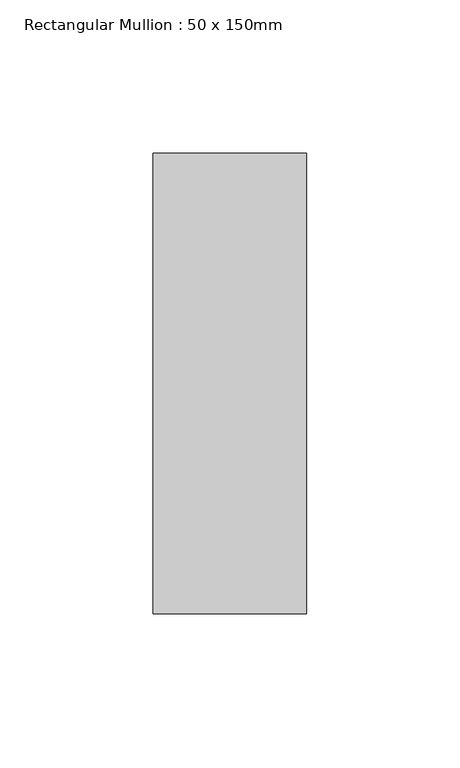
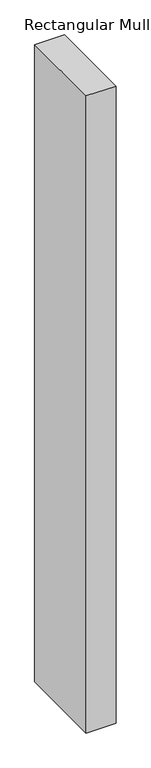
"""IFC4 building model written with IfcOpenShell, lengths in millimetres: member geometry, Rectangular Mullion : 50 x 150mm."""

from ifc_helpers import new_model, si_unit, frame, origin, place, context, project, spatial, polyline, outline, extrude, source, transform, mapped, element, save


def rectangular_mullion_50_x_150mm_abf53936(model_context):
    return source(origin(), model_context, "Body", "SweptSolid", [
        extrude(outline(polyline([(0.0, 75.0), (0.0, -75.0), (-50.0, -75.0), (-50.0, 75.0), (0.0, 75.0)])), frame((0.0, 0.0, -1133.3333333), z_axis=(0.0, 0.0, 1.0), x_axis=(1.0, 0.0, 0.0)), (0.0, 0.0, 1.0), 1133.3333333),
    ])


if __name__ == "__main__":
    model = new_model("IFC4")
    model_context = context("Model", 3, world=origin())
    ifc_project = project(units=[si_unit("LENGTHUNIT", "METRE", prefix="MILLI")], contexts=[model_context])
    site = spatial("IfcSite", under=ifc_project)
    building = spatial("IfcBuilding", under=site)
    placement = place(None, origin())
    rectangular_mullion_50_x_150mm_shape = rectangular_mullion_50_x_150mm_abf53936(model_context)
    element("IfcMember", 1, ObjectType="Rectangular Mullion : 50 x 150mm", at=placement, inside=building, context=model_context, shape_type="MappedRepresentation", body=[
        mapped(rectangular_mullion_50_x_150mm_shape, transform((0.0, 0.0, 0.0), x_axis=(1.0, 0.0, 0.0), y_axis=(0.0, 1.0, 0.0), z_axis=(0.0, 0.0, 1.0))),
    ])
    save(model, "model.ifc")

# Revit data of these elements
# Type "Rectangular Mullion : 50 x 150mm"
#   built-in parameter 1007304 = 0.492126 (stored number, unit not read)
#   built-in parameter 1007301 = 0.082021 (stored number, unit not read)
#   built-in parameter 1007300 = 0.082021 (stored number, unit not read)
# Element 1 (IfcMember, "Rectangular Mullion : 50 x 150mm")
#   Materials on its faces: "Metal - Aluminium"
# Materials
#   "Metal - Aluminium": class "Metal", colour RGB 247 247 247, transparency 0
